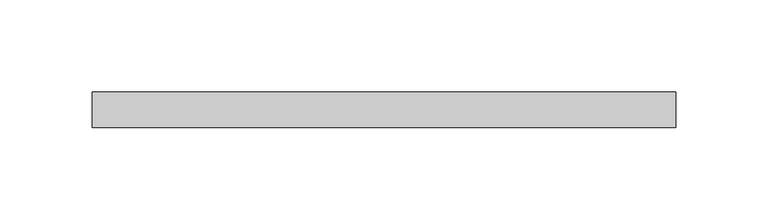
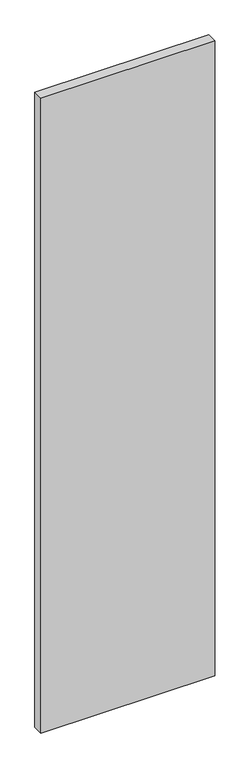
"""IFC4 building model written with IfcOpenShell, lengths in millimetres: proxy geometry, Inner panel:Inner panel:1:Inner panel:1 : Inner panel:Inner panel:300324:300043:Inner panel:1:Inner panel:1 : Inner panel:Inner panel:300324:300043 : Inner panel:Inner panel:1:Inner panel:1 : Inner panel:Inner panel:300324:300043:41 : Inner panel:Inner panel:1:Inner panel:1 : Inner panel:Inner panel:300324:300043:Inner panel:1:Inner panel:1 : Inner panel:Inner panel:300324:300043 : Inner panel:Inner panel:1:Inner panel:1 : Inner panel:Inner panel:300324:300043:300031."""

from ifc_helpers import new_model, si_unit, frame, origin, place, context, project, spatial, polyline, outline, extrude, source, transform, mapped, element, save


def generic_models_4766fb7b(model_context):
    return source(origin(), model_context, "Body", "SweptSolid", [
        extrude(outline(polyline([(667266.1522107, -568253.3163841), (667581.8275489, -568253.3163841), (667581.8275489, -568272.3663841), (667266.1522107, -568272.3663841), (667266.1522107, -568253.3163841)])), frame((0.0, 0.0, 4946.65), z_axis=(0.0, 0.0, 1.0), x_axis=(1.0, 0.0, 0.0)), (0.0, 0.0, 1.0), 1219.2),
    ])


if __name__ == "__main__":
    model = new_model("IFC4")
    model_context = context("Model", 3, world=origin())
    ifc_project = project(units=[si_unit("LENGTHUNIT", "METRE", prefix="MILLI")], contexts=[model_context])
    site = spatial("IfcSite", under=ifc_project)
    building = spatial("IfcBuilding", under=site)
    placement = place(None, origin())
    generic_models_shape = generic_models_4766fb7b(model_context)
    element("IfcBuildingElementProxy", 1, Name="Inner panel:Inner panel:1:Inner panel:1 : Inner panel:Inner panel:300324:300043:Inner panel:1:Inner panel:1 : Inner panel:Inner panel:300324:300043 : Inner panel:Inner panel:1:Inner panel:1 : Inner panel:Inner panel:300324:300043:41 : Inner panel:Inner panel:1:Inner panel:1 : Inner panel:Inner panel:300324:300043:Inner panel:1:Inner panel:1 : Inner panel:Inner panel:300324:300043 : Inner panel:Inner panel:1:Inner panel:1 : Inner panel:Inner panel:300324:300043:300031", ObjectType="Inner panel:Inner panel:1:Inner panel:1 : Inner panel:Inner panel:300324:300043:Inner panel:1:Inner panel:1 : Inner panel:Inner panel:300324:300043 : Inner panel:Inner panel:1:Inner panel:1 : Inner panel:Inner panel:300324:300043:41 : Inner panel:Inner panel:1:Inner panel:1 : Inner panel:Inner panel:300324:300043:Inner panel:1:Inner panel:1 : Inner panel:Inner panel:300324:300043 : Inner panel:Inner panel:1:Inner panel:1 : Inner panel:Inner panel:300324:300043:300031", at=placement, inside=building, context=model_context, shape_type="MappedRepresentation", body=[
        mapped(generic_models_shape, transform((0.0, 0.0, 0.0), x_axis=(1.0, 0.0, 0.0), y_axis=(0.0, 1.0, 0.0), z_axis=(0.0, 0.0, 1.0))),
    ])
    save(model, "model.ifc")

# Revit data of these elements
# Type "Inner panel:Inner panel:1:Inner panel:1 : Inner panel:Inner panel:300324:300043:Inner panel:1:Inner panel:1 : Inner panel:Inner panel:300324:300043 : Inner panel:Inner panel:1:Inner panel:1 : Inner panel:Inner panel:300324:300043:41 : Inner panel:Inner panel:1:Inner panel:1 : Inner panel:Inner panel:300324:300043:Inner panel:1:Inner panel:1 : Inner panel:Inner panel:300324:300043 : Inner panel:Inner panel:1:Inner panel:1 : Inner panel:Inner panel:300324:300043:300031"
#   NameOverride = "Inner panel:Inner panel:1:Inner panel:1 : Inner panel:Inner panel:300324:300043:Inner panel:1:Inner panel:1 : Inner panel:Inner panel:300324:300043 : Inner panel:Inner panel:1:Inner panel:1 : Inner panel:Inner panel:300324:300043:300031"
#   ObjectTypeOverride = "Inner panel:1:Inner panel:1 : Inner panel:Inner panel:300324:300043 : Inner panel:Inner panel:1:Inner panel:1 : Inner panel:Inner panel:300324:300043"
#   Reference = "Inner panel"
#   Tag = "300031"
# Element 1 (IfcBuildingElementProxy, "Inner panel:Inner panel:1:Inner panel:1 : Inner panel:Inner panel:300324:300043:Inner panel:1:Inner panel:1 : Inner panel:Inner panel:300324:300043 : Inner panel:Inner panel:1:Inner panel:1 : Inner panel:Inner panel:300324:300043:41 : Inner panel:Inner panel:1:Inner panel:1 : Inner panel:Inner panel:300324:300043:Inner panel:1:Inner panel:1 : Inner panel:Inner panel:300324:300043 : Inner panel:Inner panel:1:Inner panel:1 : Inner panel:Inner panel:300324:300043:300031")
#   Materials on its faces: "3/4\" EXTERIOR GRADE FIRE RETARDANT PLYWOOD (FINISH: GRADE B)"
# Materials
#   "3/4\" EXTERIOR GRADE FIRE RETARDANT PLYWOOD (FINISH: GRADE B)": class "Wood", colour RGB 149 120 74, transparency 0, Description = "Plywood, sheathing grade", Cost = 0
